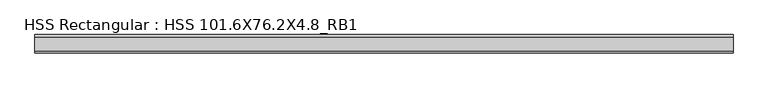
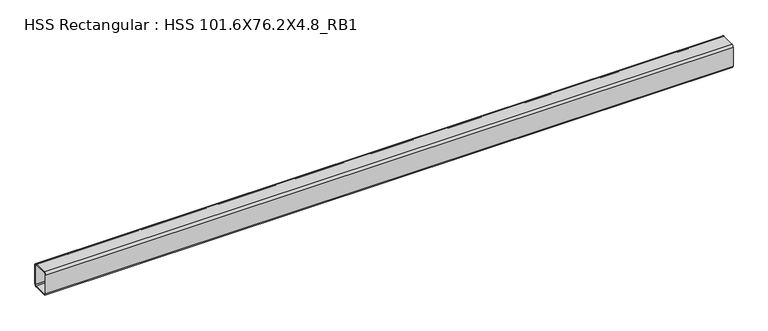
"""IFC4 building model written with IfcOpenShell, lengths in millimetres: beam geometry, HSS Rectangular : HSS 101.6X76.2X4.8_RB1."""

from ifc_helpers import new_model, si_unit, point, frame, frame_2d, origin, place, context, project, spatial, polyline, circle_curve, trimmed, segment, composite_curve, outline, extrude, source, transform, mapped, element, save


def hss_rectangular_hss_101_6x76_2x4_8_rb1_bafa1cf1(model_context):
    return source(origin(), model_context, "Body", "SweptSolid", [
        extrude(outline(composite_curve([segment(polyline([(38.1, 41.275), (38.1, -41.275)]), True, "CONTINUOUS"), segment(trimmed(circle_curve(frame_2d((28.575, -41.275)), 9.525), [point((38.1, -41.275))], [point((28.575, -50.8))], False, "CARTESIAN"), True, "CONTINUOUS"), segment(polyline([(28.575, -50.8), (-28.575, -50.8)]), True, "CONTINUOUS"), segment(trimmed(circle_curve(frame_2d((-28.575, -41.275)), 9.525), [point((-28.575, -50.8))], [point((-38.1, -41.275))], False, "CARTESIAN"), True, "CONTINUOUS"), segment(polyline([(-38.1, -41.275), (-38.1, 41.275)]), True, "CONTINUOUS"), segment(trimmed(circle_curve(frame_2d((-28.575, 41.275)), 9.525), [point((-38.1, 41.275))], [point((-28.575, 50.8))], False, "CARTESIAN"), True, "CONTINUOUS"), segment(polyline([(-28.575, 50.8), (28.575, 50.8)]), True, "CONTINUOUS"), segment(trimmed(circle_curve(frame_2d((28.575, 41.275)), 9.525), [point((28.575, 50.8))], [point((38.1, 41.275))], False, "CARTESIAN"), True, "CONTINUOUS")], self_intersect=False), holes=[composite_curve([segment(trimmed(circle_curve(frame_2d((-28.575, 41.275)), 4.7625), [point((-28.575, 46.0375))], [point((-33.3375, 41.275))], True, "CARTESIAN"), True, "CONTINUOUS"), segment(polyline([(-33.3375, 41.275), (-33.3375, -41.275)]), True, "CONTINUOUS"), segment(trimmed(circle_curve(frame_2d((-28.575, -41.275)), 4.7625), [point((-33.3375, -41.275))], [point((-28.575, -46.0375))], True, "CARTESIAN"), True, "CONTINUOUS"), segment(polyline([(-28.575, -46.0375), (28.575, -46.0375)]), True, "CONTINUOUS"), segment(trimmed(circle_curve(frame_2d((28.575, -41.275)), 4.7625), [point((28.575, -46.0375))], [point((33.3375, -41.275))], True, "CARTESIAN"), True, "CONTINUOUS"), segment(polyline([(33.3375, -41.275), (33.3375, 41.275)]), True, "CONTINUOUS"), segment(trimmed(circle_curve(frame_2d((28.575, 41.275)), 4.7625), [point((33.3375, 41.275))], [point((28.575, 46.0375))], True, "CARTESIAN"), True, "CONTINUOUS"), segment(polyline([(28.575, 46.0375), (-28.575, 46.0375)]), True, "CONTINUOUS")], self_intersect=False)]), frame((-1442.3750006, 0.0, 0.0), z_axis=(1.0, 0.0, 0.0), x_axis=(0.0, 1.0, 0.0)), (0.0, 0.0, 1.0), 2884.7500012),
    ])


if __name__ == "__main__":
    model = new_model("IFC4")
    model_context = context("Model", 3, world=origin())
    ifc_project = project(units=[si_unit("LENGTHUNIT", "METRE", prefix="MILLI")], contexts=[model_context])
    site = spatial("IfcSite", under=ifc_project)
    building = spatial("IfcBuilding", under=site)
    placement = place(None, origin())
    hss_rectangular_hss_101_6x76_2x4_8_rb1_shape = hss_rectangular_hss_101_6x76_2x4_8_rb1_bafa1cf1(model_context)
    element("IfcBeam", 1, ObjectType="HSS Rectangular : HSS 101.6X76.2X4.8_RB1", at=placement, inside=building, context=model_context, shape_type="MappedRepresentation", body=[
        mapped(hss_rectangular_hss_101_6x76_2x4_8_rb1_shape, transform((0.0, 0.0, 0.0), x_axis=(1.0, 0.0, 0.0), y_axis=(0.0, 1.0, 0.0), z_axis=(0.0, 0.0, 1.0))),
    ])
    save(model, "model.ifc")

# Revit data of these elements
# Type "HSS Rectangular : HSS 101.6X76.2X4.8_RB1"
#   Section Name Key = "HSS 4X3X3/16"
#   Assembly Code = "B10"
#   Width = 7.62 cm
#   Wall Nominal Thickness = 0.4763 cm
#   Wall Design Thickness = 0.442 cm
#   Torsional Moment of Inertia = 260.561 cm⁴
#   Torsional Modulus = 61.2876 cm³
#   Section Area = 14.4516 cm²
#   Plastic Modulus weak axis = 40.3122 cm³
#   Plastic Modulus strong axis = 49.1612 cm³
#   Perimeter = 0.881482 m²/m
#   Outer Fillet = 0.9525 cm
#   Nominal Weight = 12.1285 kgf/m
#   Moment of Inertia weak axis = 131.529 cm⁴
#   Moment of Inertia strong axis = 205.202 cm⁴
#   Inner Fillet = 0.4763 cm
#   Height = 10.16 cm
#   Elastic Modulus weak axis = 34.4128 cm³
#   Elastic Modulus strong axis = 40.476 cm³
#   Centroid Vertical = 5.08 cm
#   Centroid Horizontal = 3.81 cm
#   Length [instance default] = 1524 mm
#   Structural Material [instance default] = Steel ASTM A500, Grade B, Rectangular and Square
#   Principal Axes Angle = 0
# Element 1 (IfcBeam, "HSS Rectangular : HSS 101.6X76.2X4.8_RB1")
#   Structural Material = Steel ASTM A992
#   Materials on its faces: "Steel ASTM A992"
# Materials
#   "Steel ASTM A500, Grade B, Rectangular and Square": class "Metal", colour RGB 199 199 199, transparency 0, Description = "Carbon steel", Cost = 0
#   "Steel ASTM A992": class "Metal", colour RGB 199 199 199, transparency 0, Description = "Structural steel 50ksi", Cost = 0
